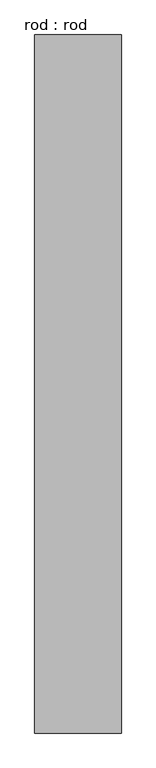
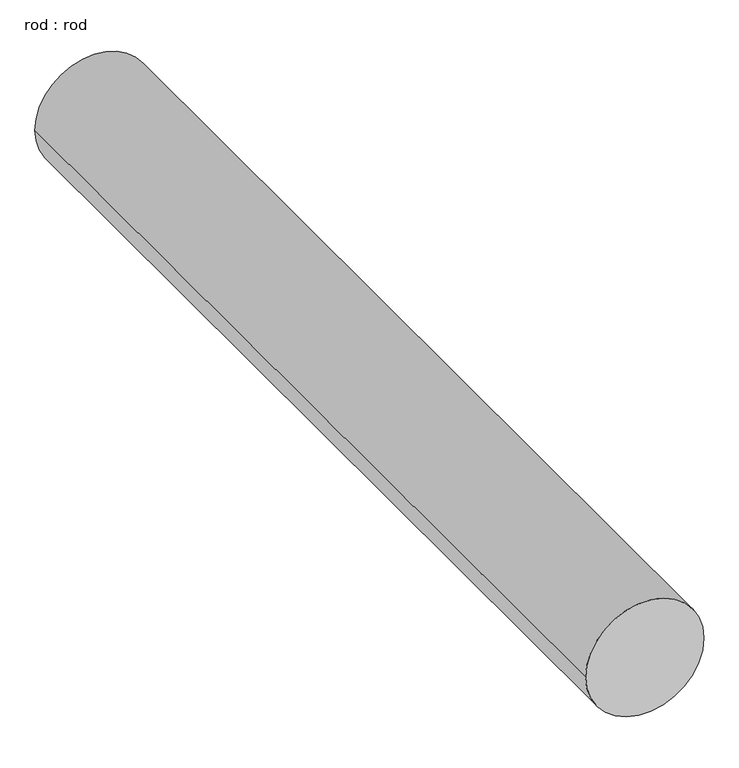
"""IFC4 building model written with IfcOpenShell, lengths in millimetres: proxy geometry, rod : rod."""

from ifc_helpers import new_model, si_unit, point, frame, frame_2d, origin, place, context, project, spatial, circle_curve, trimmed, segment, composite_curve, outline, extrude, source, transform, mapped, element, save


def rod_rod_dafd0e36(model_context):
    return source(origin(), model_context, "Body", "SweptSolid", [
        extrude(outline(composite_curve([segment(trimmed(circle_curve(frame_2d((0.0108462, 0.0)), 200.0), [point((0.0108462, 200.0))], [point((0.0108462, -200.0))], False, "CARTESIAN"), True, "CONTINUOUS"), segment(trimmed(circle_curve(frame_2d((0.0108462, 0.0)), 200.0), [point((0.0108462, -200.0))], [point((0.0108462, 200.0))], False, "CARTESIAN"), True, "CONTINUOUS")], self_intersect=False)), frame((0.0, 2480.2286153, 0.0), z_axis=(0.0, 1.0, 0.0), x_axis=(0.0, 0.0, 1.0)), (0.0, 0.0, 1.0), 3225.0),
    ])


if __name__ == "__main__":
    model = new_model("IFC4")
    model_context = context("Model", 3, world=origin())
    ifc_project = project(units=[si_unit("LENGTHUNIT", "METRE", prefix="MILLI")], contexts=[model_context])
    site = spatial("IfcSite", under=ifc_project)
    building = spatial("IfcBuilding", under=site)
    placement = place(None, origin())
    rod_rod_shape = rod_rod_dafd0e36(model_context)
    element("IfcBuildingElementProxy", 1, Name="rod : rod", ObjectType="rod : rod", at=placement, inside=building, context=model_context, shape_type="MappedRepresentation", body=[
        mapped(rod_rod_shape, transform((0.0, 0.0, 0.0), x_axis=(1.0, 0.0, 0.0), y_axis=(0.0, 1.0, 0.0), z_axis=(0.0, 0.0, 1.0))),
    ])
    save(model, "model.ifc")

# Revit data of these elements
# Type "rod : rod"
#   Default Elevation = 0
